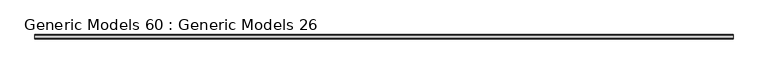
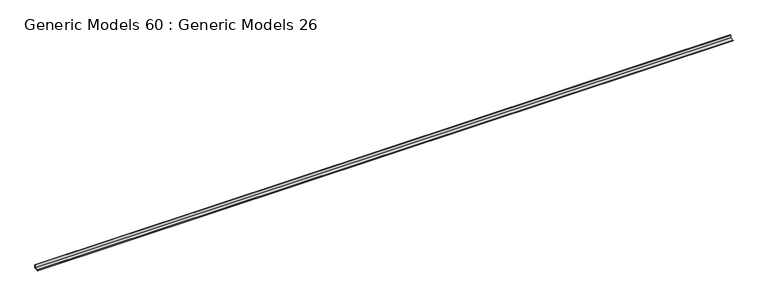
"""IFC4 building model written with IfcOpenShell, lengths in millimetres: proxy geometry, Generic Models 60 : Generic Models 26."""

from ifc_helpers import new_model, si_unit, frame, origin, place, context, project, spatial, polyline, outline, extrude, source, transform, mapped, element, save


def generic_models_60_generic_models_26_15c3100d(model_context):
    return source(origin(), model_context, "Body", "SweptSolid", [
        extrude(outline(polyline([(25532.5071923, 269266.1659555), (25498.9890229, 269266.1659555), (25494.4988948, 269261.6758275), (25493.3763628, 269262.7983595), (25498.3314588, 269267.7534555), (25530.9196923, 269267.7534555), (25530.9196923, 269294.4089862), (25532.5071923, 269294.4089862), (25532.5071923, 269266.1659555)])), frame((27760.6090778, 0.0, 0.0), z_axis=(1.0, 0.0, 0.0), x_axis=(0.0, 1.0, 0.0)), (0.0, 0.0, 1.0), 6032.7256636),
    ])


if __name__ == "__main__":
    model = new_model("IFC4")
    model_context = context("Model", 3, world=origin())
    ifc_project = project(units=[si_unit("LENGTHUNIT", "METRE", prefix="MILLI")], contexts=[model_context])
    site = spatial("IfcSite", under=ifc_project)
    building = spatial("IfcBuilding", under=site)
    placement = place(None, origin())
    generic_models_60_generic_models_26_shape = generic_models_60_generic_models_26_15c3100d(model_context)
    element("IfcBuildingElementProxy", 1, Name="Generic Models 60 : Generic Models 26", ObjectType="Generic Models 60 : Generic Models 26", at=placement, inside=building, context=model_context, shape_type="MappedRepresentation", body=[
        mapped(generic_models_60_generic_models_26_shape, transform((0.0, 0.0, 0.0), x_axis=(1.0, 0.0, 0.0), y_axis=(0.0, 1.0, 0.0), z_axis=(0.0, 0.0, 1.0))),
    ])
    save(model, "model.ifc")

# Revit data of these elements
# Element 1 (IfcBuildingElementProxy, "Generic Models 60 : Generic Models 26")
#   Materials on its faces: "GALV. BRAKE METAL - (COLOR: GALV.)"
# Materials
#   "GALV. BRAKE METAL - (COLOR: GALV.)": class "Generic", colour RGB 234 234 234, transparency 0, Cost = 0
